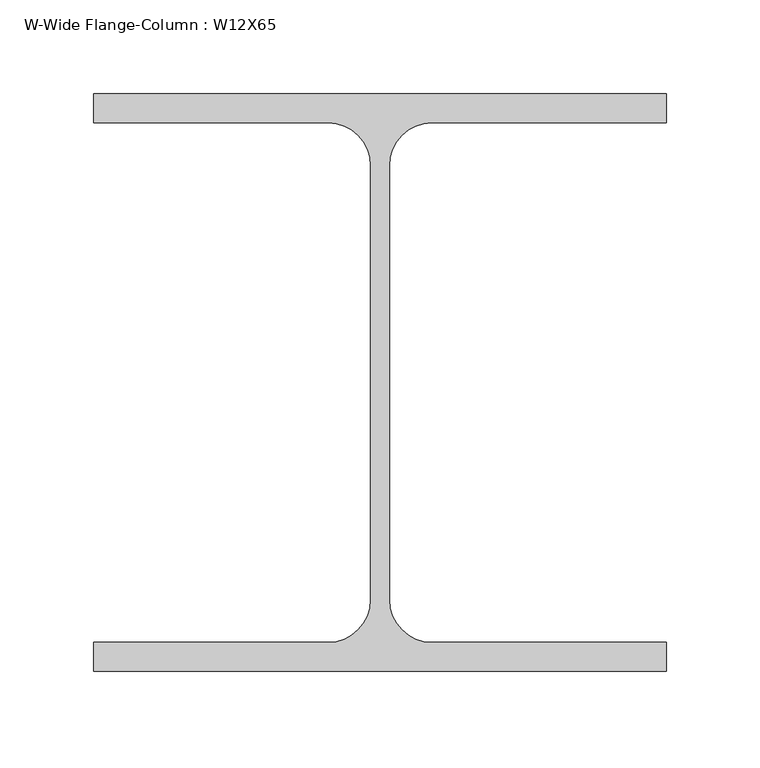
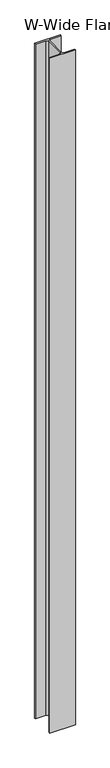
"""IFC4 building model written with IfcOpenShell, lengths in millimetres: column geometry, W-Wide Flange-Column : W12X65."""

from ifc_helpers import new_model, si_unit, point, frame, frame_2d, origin, place, context, project, spatial, polyline, circle_curve, trimmed, segment, composite_curve, outline, extrude, source, transform, mapped, element, save


def w_wide_flange_column_w12x65_dbb9e44c(model_context):
    return source(origin(), model_context, "Body", "SweptSolid", [
        extrude(outline(composite_curve([segment(polyline([(152.4, 153.67), (152.4, 138.303), (27.686, 138.303)]), True, "CONTINUOUS"), segment(trimmed(circle_curve(frame_2d((27.686, 115.57)), 22.733), [point((27.686, 138.303))], [point((4.953, 115.57))], True, "CARTESIAN"), True, "CONTINUOUS"), segment(polyline([(4.953, 115.57), (4.953, -115.57)]), True, "CONTINUOUS"), segment(trimmed(circle_curve(frame_2d((27.686, -115.57)), 22.733), [point((4.953, -115.57))], [point((27.686, -138.303))], True, "CARTESIAN"), True, "CONTINUOUS"), segment(polyline([(27.686, -138.303), (152.4, -138.303), (152.4, -153.67), (-152.4, -153.67), (-152.4, -138.303), (-27.686, -138.303)]), True, "CONTINUOUS"), segment(trimmed(circle_curve(frame_2d((-27.686, -115.57)), 22.733), [point((-27.686, -138.303))], [point((-4.953, -115.57))], True, "CARTESIAN"), True, "CONTINUOUS"), segment(polyline([(-4.953, -115.57), (-4.953, 115.57)]), True, "CONTINUOUS"), segment(trimmed(circle_curve(frame_2d((-27.686, 115.57)), 22.733), [point((-4.953, 115.57))], [point((-27.686, 138.303))], True, "CARTESIAN"), True, "CONTINUOUS"), segment(polyline([(-27.686, 138.303), (-152.4, 138.303), (-152.4, 153.67), (152.4, 153.67)]), True, "CONTINUOUS")], self_intersect=False)), frame((0.0, 0.0, 9163.05), z_axis=(0.0, 0.0, 1.0), x_axis=(1.0, 0.0, 0.0)), (0.0, 0.0, 1.0), 8464.55),
    ])


if __name__ == "__main__":
    model = new_model("IFC4")
    model_context = context("Model", 3, world=origin())
    ifc_project = project(units=[si_unit("LENGTHUNIT", "METRE", prefix="MILLI")], contexts=[model_context])
    site = spatial("IfcSite", under=ifc_project)
    building = spatial("IfcBuilding", under=site)
    placement = place(None, origin())
    w_wide_flange_column_w12x65_shape = w_wide_flange_column_w12x65_dbb9e44c(model_context)
    element("IfcColumn", 1, ObjectType="W-Wide Flange-Column : W12X65", at=placement, inside=building, context=model_context, shape_type="MappedRepresentation", body=[
        mapped(w_wide_flange_column_w12x65_shape, transform((0.0, 0.0, 0.0), x_axis=(1.0, 0.0, 0.0), y_axis=(0.0, 1.0, 0.0), z_axis=(0.0, 0.0, 1.0))),
    ])
    save(model, "model.ifc")

# Revit data of these elements
# Type "W-Wide Flange-Column : W12X65"
#   Assembly Code = "B10"
#   W = 65
#   bf = 1' - 0"
#   d = 1' - 0.1"
#   k = 0' - 1 1/2"
#   kr = 0' - 0.895"
#   tf = 0' - 0.605"
#   tw = 0' - 0.39"
#   A = 0.132639 SF
#   Structural Material [instance default] = Steel ASTM A992
# Element 1 (IfcColumn, "W-Wide Flange-Column : W12X65")
#   Materials on its faces: "Steel ASTM A992"
# Materials
#   "Steel ASTM A992": class "Metal", colour RGB 199 199 199, transparency 0, Description = "Structural steel 50ksi", Cost = 0
